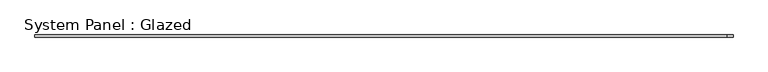
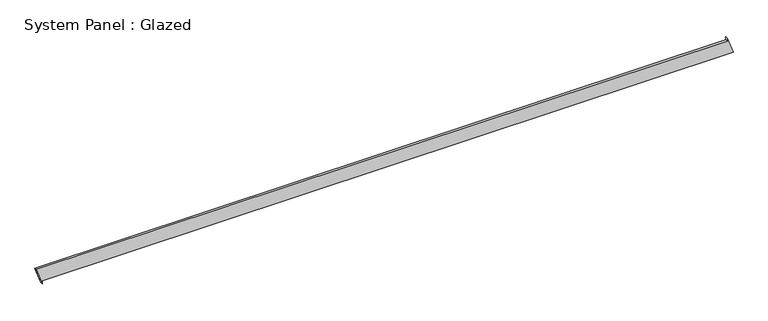
"""IFC4 building model written with IfcOpenShell, lengths in millimetres: plate geometry, System Panel : Glazed."""

from ifc_helpers import new_model, si_unit, frame, origin, place, context, project, spatial, polyline, outline, extrude, source, transform, mapped, element, save


def system_panel_glazed_45afaa7f(model_context):
    return source(origin(), model_context, "Body", "SweptSolid", [
        extrude(outline(polyline([(0.0, -3959.3834758), (35.3553391, -3959.3834758), (35.3553391, 4028.0417319), (234.7714122, 3959.4163917), (199.4160731, 3959.4164519), (199.4024711, -4028.0417319), (0.0, -3959.3834758)])), frame((0.0, -49.5, 0.0), z_axis=(0.0, 1.0, 0.0), x_axis=(0.0, 0.0, 1.0)), (0.0, 0.0, 1.0), 25.0),
    ])


if __name__ == "__main__":
    model = new_model("IFC4")
    model_context = context("Model", 3, world=origin())
    ifc_project = project(units=[si_unit("LENGTHUNIT", "METRE", prefix="MILLI")], contexts=[model_context])
    site = spatial("IfcSite", under=ifc_project)
    building = spatial("IfcBuilding", under=site)
    placement = place(None, origin())
    system_panel_glazed_shape = system_panel_glazed_45afaa7f(model_context)
    element("IfcPlate", 1, ObjectType="System Panel : Glazed", at=placement, inside=building, context=model_context, shape_type="MappedRepresentation", body=[
        mapped(system_panel_glazed_shape, transform((0.0, 0.0, 0.0), x_axis=(1.0, 0.0, 0.0), y_axis=(0.0, 1.0, 0.0), z_axis=(0.0, 0.0, 1.0))),
    ])
    save(model, "model.ifc")

# Revit data of these elements
# Element 1 (IfcPlate, "System Panel : Glazed")
#   Materials on its faces: "Glass"
# Materials
#   "Glass": class "Glass", colour RGB 218 227 224, transparency 0.85, Description = "Soda Lime Glass", Cost = 0
